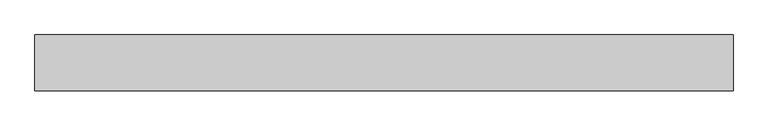
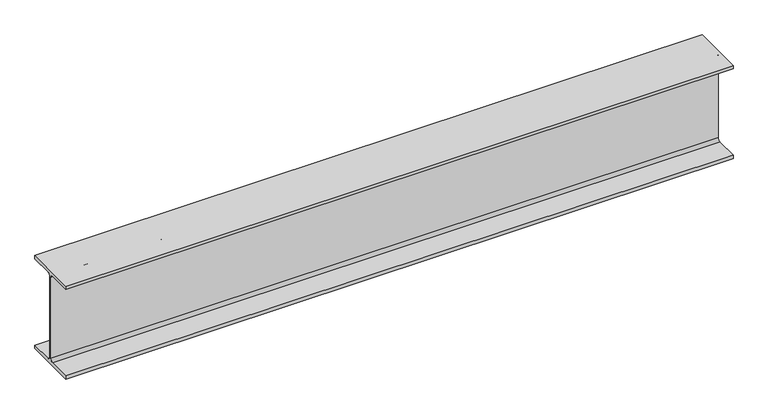
"""IFC4 building model written with IfcOpenShell, lengths in millimetres: beam geometry, Steel Beam_H-KSD3502 : H_SB_ASB_H-194x150x6x9."""

from ifc_helpers import new_model, si_unit, point, frame, frame_2d, origin, place, context, project, spatial, polyline, circle_curve, trimmed, segment, composite_curve, outline, extrude, source, transform, mapped, element, save


def beam_ff7b883b(model_context):
    return source(origin(), model_context, "Body", "SweptSolid", [
        extrude(outline(composite_curve([segment(polyline([(-82.5, -141.5), (-11.9, -141.5)]), True, "CONTINUOUS"), segment(trimmed(circle_curve(frame_2d((-11.9, -132.6)), 8.9), [point((-11.9, -141.5))], [point((-3.0, -132.6))], True, "CARTESIAN"), True, "CONTINUOUS"), segment(polyline([(-3.0, -132.6), (-3.0, 132.6)]), True, "CONTINUOUS"), segment(trimmed(circle_curve(frame_2d((-11.9, 132.6)), 8.9), [point((-3.0, 132.6))], [point((-11.9, 141.5))], True, "CARTESIAN"), True, "CONTINUOUS"), segment(polyline([(-11.9, 141.5), (-82.5, 141.5), (-82.5, 151.7), (82.5, 151.7), (82.5, 141.5), (11.9, 141.5)]), True, "CONTINUOUS"), segment(trimmed(circle_curve(frame_2d((11.9, 132.6)), 8.9), [point((11.9, 141.5))], [point((3.0, 132.6))], True, "CARTESIAN"), True, "CONTINUOUS"), segment(polyline([(3.0, 132.6), (3.0, -132.6)]), True, "CONTINUOUS"), segment(trimmed(circle_curve(frame_2d((11.9, -132.6)), 8.9), [point((3.0, -132.6))], [point((11.9, -141.5))], True, "CARTESIAN"), True, "CONTINUOUS"), segment(polyline([(11.9, -141.5), (82.5, -141.5), (82.5, -151.7), (-82.5, -151.7), (-82.5, -141.5)]), True, "CONTINUOUS")], self_intersect=False)), frame((-1171.2564634, 0.0, 0.0), z_axis=(1.0, 0.0, 0.0), x_axis=(0.0, 1.0, 0.0)), (0.0, 0.0, 1.0), 2060.1030758),
    ])


if __name__ == "__main__":
    model = new_model("IFC4")
    model_context = context("Model", 3, world=origin())
    ifc_project = project(units=[si_unit("LENGTHUNIT", "METRE", prefix="MILLI")], contexts=[model_context])
    site = spatial("IfcSite", under=ifc_project)
    building = spatial("IfcBuilding", under=site)
    placement = place(None, origin())
    beam_shape = beam_ff7b883b(model_context)
    element("IfcBeam", 1, ObjectType="Steel Beam_H-KSD3502 : H_SB_ASB_H-194x150x6x9", at=placement, inside=building, context=model_context, shape_type="MappedRepresentation", body=[
        mapped(beam_shape, transform((0.0, 0.0, 0.0), x_axis=(1.0, 0.0, 0.0), y_axis=(0.0, 1.0, 0.0), z_axis=(0.0, 0.0, 1.0))),
    ])
    save(model, "model.ifc")

# Revit data of these elements
# Type "Steel Beam_H-KSD3502 : H_SB_ASB_H-194x150x6x9"
#   Width = 15.0 cm
#   Web Thickness = 0.6 cm
#   Web Fillet = 1.3 cm
#   Warping Constant = 43316.0 cm⁶
#   Torsional Moment of Inertia = 8.622 cm⁴
#   Torsional Modulus = 1.0 cm³
#   Section Area = 39.01 cm²
#   Plastic Modulus weak axis = 104.0 cm³
#   Plastic Modulus strong axis = 309.0 cm³
#   Perimeter = 0.95 m²/m
#   Nominal Weight = 30.60 kgf/m
#   Moment of Inertia weak axis = 507.00 cm⁴
#   Moment of Inertia strong axis = 2690.00 cm⁴
#   Height = 19.4 cm
#   Flange Thickness = 0.9 cm
#   Elastic Modulus weak axis = 67.6 cm³
#   Elastic Modulus strong axis = 277.0 cm³
#   Centroid Vertical = 9.7 cm
#   Centroid Horizontal = 7.5 cm
#   Length [instance default] = 1.5240 m
#   Structural Material [instance default] = Steel, 45-345
#   Assembly Code = ""
# Element 1 (IfcBeam, "Steel Beam_H-KSD3502 : H_SB_ASB_H-194x150x6x9")
#   Structural Material = none
# Materials
#   "Steel, 45-345": class "Metal", colour RGB 189 187 185, transparency 0, Description = "Steel 345 MPa", Cost = 0
